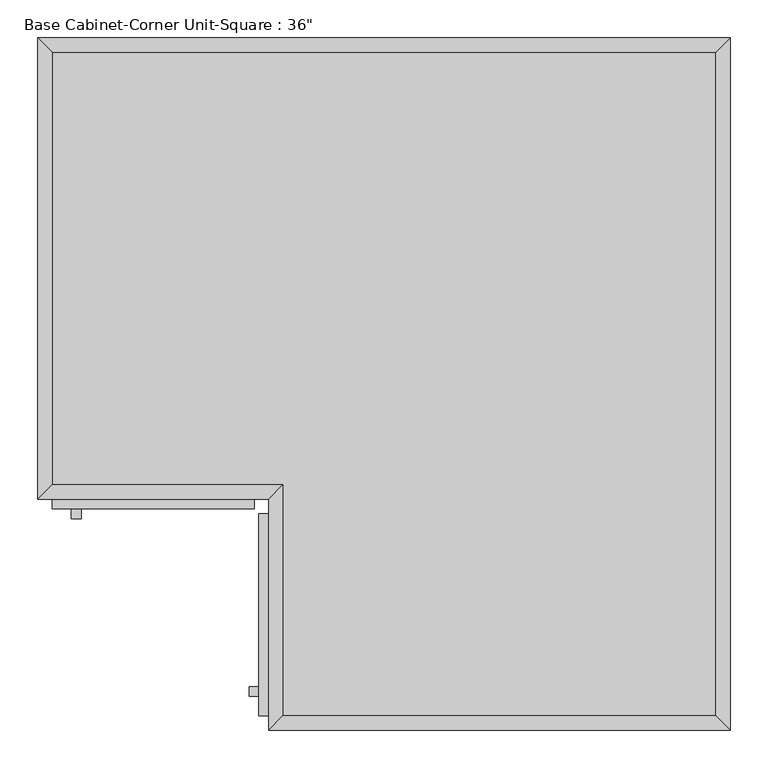
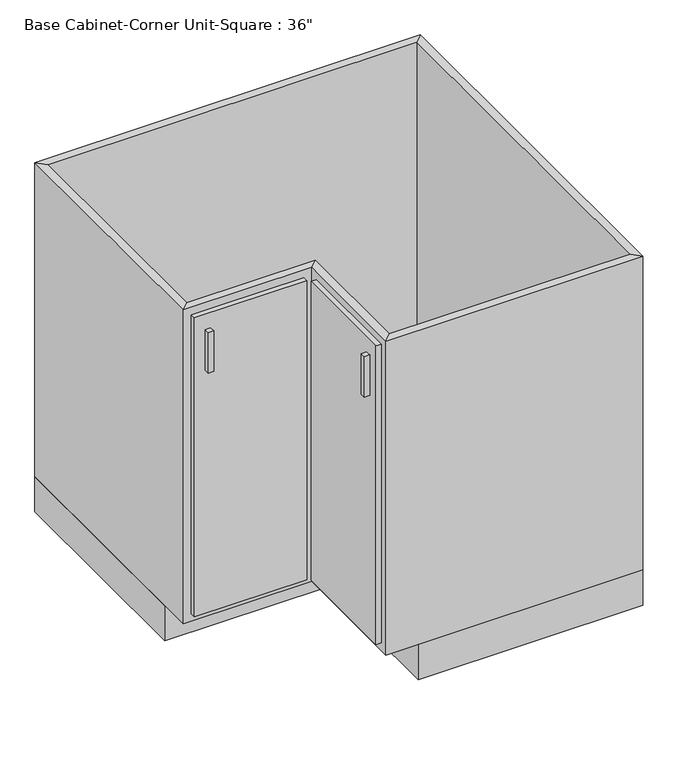
"""IFC4 building model written with IfcOpenShell, lengths in millimetres: furniture geometry."""

from ifc_helpers import new_model, si_unit, frame, origin, origin_with_axes, place, context, project, spatial, polyline, outline, extrude, faceted_brep, source, transform, mapped, element, save


def furniture_24324f2d(model_context):
    return source(origin(), model_context, "Body", "SolidModel", [
        extrude(outline(polyline([(-95.5622951, -857.25), (-95.5622951, -869.95), (-108.2622951, -869.95), (-108.2622951, -857.25), (-95.5622951, -857.25)])), frame((0.0, 0.0, 717.55), z_axis=(0.0, 0.0, 1.0), x_axis=(1.0, 0.0, 0.0)), (0.0, 0.0, 1.0), 101.6),
        extrude(outline(polyline([(-82.8622951, -628.65), (-82.8622951, -895.35), (-95.5622951, -895.35), (-95.5622951, -628.65), (-82.8622951, -628.65)])), frame((0.0, 0.0, 107.95), z_axis=(0.0, 0.0, 1.0), x_axis=(1.0, 0.0, 0.0)), (0.0, 0.0, 1.0), 749.3),
        extrude(outline(polyline([(-330.5122951, -635.0), (-343.2122951, -635.0), (-343.2122951, -622.3), (-330.5122951, -622.3), (-330.5122951, -635.0)])), frame((0.0, 0.0, 717.55), z_axis=(0.0, 0.0, 1.0), x_axis=(1.0, 0.0, 0.0)), (0.0, 0.0, 1.0), 101.6),
        extrude(outline(polyline([(-101.9122951, -622.3), (-368.6122951, -622.3), (-368.6122951, -609.6), (-101.9122951, -609.6), (-101.9122951, -622.3)])), frame((0.0, 0.0, 107.95), z_axis=(0.0, 0.0, 1.0), x_axis=(1.0, 0.0, 0.0)), (0.0, 0.0, 1.0), 749.3),
        faceted_brep([(507.6877049, -895.35, 876.3), (507.6877049, -895.35, 88.9), (-63.8122951, -895.35, 88.9), (-63.8122951, -895.35, 876.3), (526.7377049, -914.4, 876.3), (-82.8622951, -914.4, 876.3), (526.7377049, -914.4, 88.9), (-82.8622951, -914.4, 88.9), (-63.8122951, -590.55, 88.9), (-63.8122951, -590.55, 876.3), (-82.8622951, -609.6, 876.3), (-82.8622951, -609.6, 88.9), (-368.6122951, -590.55, 88.9), (-368.6122951, -590.55, 876.3), (-387.6622951, -609.6, 876.3), (-387.6622951, -609.6, 88.9), (-368.6122951, -19.05, 88.9), (-368.6122951, -19.05, 876.3), (-387.6622951, 0.0, 876.3), (-387.6622951, 0.0, 88.9), (507.6877049, -19.05, 88.9), (507.6877049, -19.05, 876.3), (526.7377049, 0.0, 876.3), (526.7377049, 0.0, 88.9)], [[[0, 1, 2, 3]], [[4, 0, 3, 5]], [[6, 4, 5, 7]], [[1, 6, 7, 2]], [[3, 2, 8, 9]], [[5, 3, 9, 10]], [[7, 5, 10, 11]], [[2, 7, 11, 8]], [[9, 8, 12, 13]], [[10, 9, 13, 14]], [[11, 10, 14, 15]], [[8, 11, 15, 12]], [[13, 12, 16, 17]], [[14, 13, 17, 18]], [[15, 14, 18, 19]], [[12, 15, 19, 16]], [[17, 16, 20, 21]], [[18, 17, 21, 22]], [[19, 18, 22, 23]], [[16, 19, 23, 20]], [[21, 20, 1, 0]], [[22, 21, 0, 4]], [[23, 22, 4, 6]], [[20, 23, 6, 1]]]),
        extrude(outline(polyline([(507.6877049, -19.05), (507.6877049, -895.35), (-63.8122951, -895.35), (-63.8122951, -590.55), (-368.6122951, -590.55), (-368.6122951, -19.05), (507.6877049, -19.05)])), frame((0.0, 0.0, 88.9), z_axis=(0.0, 0.0, 1.0), x_axis=(1.0, 0.0, 0.0)), (0.0, 0.0, 1.0), 19.05),
        extrude(outline(polyline([(526.7377049, 0.0), (526.7377049, -914.4), (-6.6622951, -914.4), (-6.6622951, -533.4), (-387.6622951, -533.4), (-387.6622951, 0.0), (526.7377049, 0.0)])), origin_with_axes(), (0.0, 0.0, 1.0), 88.9),
    ])


if __name__ == "__main__":
    model = new_model("IFC4")
    model_context = context("Model", 3, world=origin())
    ifc_project = project(units=[si_unit("LENGTHUNIT", "METRE", prefix="MILLI")], contexts=[model_context])
    site = spatial("IfcSite", under=ifc_project)
    building = spatial("IfcBuilding", under=site)
    placement = place(None, origin())
    furniture_shape = furniture_24324f2d(model_context)
    element("IfcFurniture", 1, ObjectType="Base Cabinet-Corner Unit-Square : 36\"", at=placement, inside=building, context=model_context, shape_type="MappedRepresentation", body=[
        mapped(furniture_shape, transform((0.0, 0.0, 0.0), x_axis=(1.0, 0.0, 0.0), y_axis=(0.0, 1.0, 0.0), z_axis=(0.0, 0.0, 1.0))),
    ])
    save(model, "model.ifc")

# Revit data of these elements
# Type "Base Cabinet-Corner Unit-Square : 36\""
#   COBie.Type.CreatedBy = "doug.wood@us.ibm.com"
#   COBie.Type.CreatedOn = "2016-04-14T02:14:45"
#   COBie.Type.Name = "Casework_Base Cabinet-Corner Unit-Square_36\""
#   COBie.Type.Category = "C1030410"
#   COBie.Type.Description = "Base Cabinet-Corner Unit-Square_36\""
#   COBie.Type.Manufacturer = ""
#   COBie.Type.ModelNumber = ""
#   Assembly Code = "C1030410"
#   COBie.Type.ReplacementCost = 0
#   Depth = 2' - 0"
#   Height = 2' - 10 1/2"
#   Toe Depth = 0' - 3"
#   Toe Height = 0' - 3 1/2"
#   Width = 3' - 0"
#   COBie.Type = no
#   Cabinet Material = Cabinets
#   Door/Drawer Material = Cabinets
#   Handle Material = Cabinets - Handles
# Element 1 (IfcFurniture, "Base Cabinet-Corner Unit-Square : 36\"")
#   Materials on its faces: "Cabinets", "Cabinets - Handles"
# Materials
#   "Cabinets": class "Miscellaneous", colour RGB 249 249 249, transparency 0
#   "Cabinets - Handles": class "Metal", colour RGB 57 57 57, transparency 0
